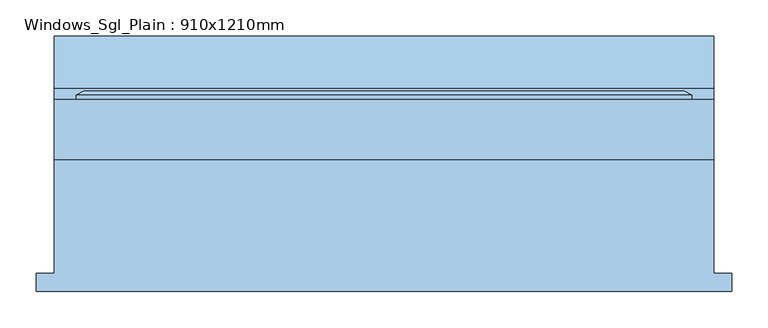
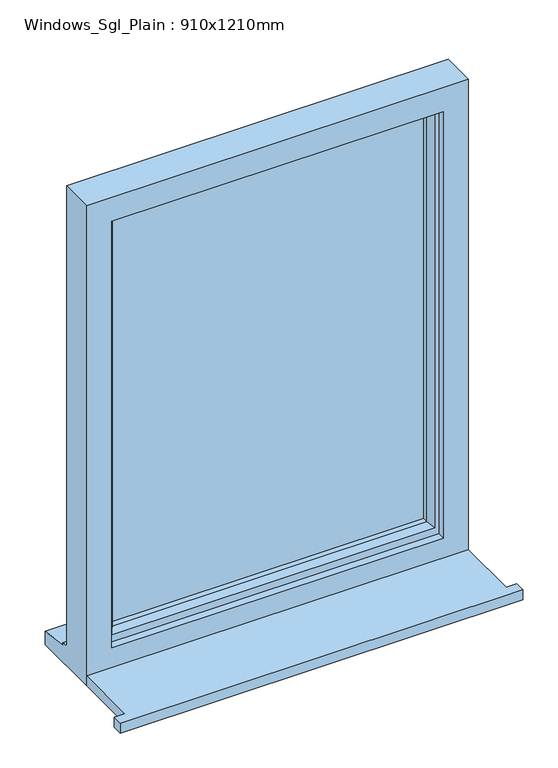
"""IFC4 building model written with IfcOpenShell, lengths in millimetres: window geometry, Windows_Sgl_Plain : 910x1210mm."""

import ifcopenshell
import ifcopenshell.guid

model = None  # the IFC model being written
_history = None  # IfcOwnerHistory: only IFC2X3 demands one
_inside = {}  # id of a spatial element -> (the spatial element, [elements in it])
_under = {}  # id of a project, library or spatial element -> (it, [spatial elements below it])
_declared = {}  # id of a project -> (the project, [libraries it declares])
_typed = {}  # id of a type object -> (the type object, [elements of that type])
_made_of = {}  # id of a material, layer set ... -> (it, [elements and type objects made of it])


def new_model(schema):
    """Start an empty IFC model of exactly this schema.

    Asked for "IFC4X3", IfcOpenShell would pick the latest addendum, in which some entities
    have other attributes; the version numbers below select the first issue.
    IFC2X3 requires an IfcOwnerHistory on every rooted entity: one is made here for all.
    """
    global model, _history
    if schema == "IFC4X3":
        model = ifcopenshell.file(schema_version=(4, 3, 0, 0))
    else:
        model = ifcopenshell.file(schema=schema)
    _inside.clear()
    _under.clear()
    _declared.clear()
    _typed.clear()
    _made_of.clear()
    _history = None
    if model.schema == "IFC2X3":
        org = make("IfcOrganization", Name="unknown")
        user = make(
            "IfcPersonAndOrganization",
            ThePerson=make("IfcPerson", FamilyName="unknown"),
            TheOrganization=org,
        )
        app = make(
            "IfcApplication",
            ApplicationDeveloper=org,
            Version="unknown",
            ApplicationFullName="unknown",
            ApplicationIdentifier="unknown",
        )
        _history = make(
            "IfcOwnerHistory",
            OwningUser=user,
            OwningApplication=app,
            ChangeAction="ADDED",
            CreationDate=0,
        )
    return model


def make(cls, **values):
    """One entity of the class cls with the attributes given. An attribute that is None is left unset."""
    return model.create_entity(
        cls, **{name: value for name, value in values.items() if value is not None}
    )


def rooted(cls, **values):
    """An entity with a GlobalId (a new one), such as an element, a storey or a relation."""
    return make(cls, GlobalId=ifcopenshell.guid.new(), OwnerHistory=_history, **values)


def si_unit(unit_type, name, prefix=None):
    """IfcSIUnit, for example si_unit("LENGTHUNIT", "METRE", prefix="MILLI")."""
    return make("IfcSIUnit", UnitType=unit_type, Prefix=prefix, Name=name)


def assignment(units):
    """IfcUnitAssignment: the units of a project."""
    return None if units is None else make("IfcUnitAssignment", Units=units)


def point(xyz):
    """IfcCartesianPoint."""
    return None if xyz is None else make("IfcCartesianPoint", Coordinates=xyz)


def direction(xyz):
    """IfcDirection."""
    return None if xyz is None else make("IfcDirection", DirectionRatios=xyz)


def frame(location, z_axis=None, x_axis=None):
    """IfcAxis2Placement3D, a coordinate frame: its origin and axes. An axis left out is left unset."""
    return make(
        "IfcAxis2Placement3D",
        Location=point(location),
        Axis=direction(z_axis),
        RefDirection=direction(x_axis),
    )


def origin():
    """The frame at (0, 0, 0) with its axes left unset."""
    return frame((0.0, 0.0, 0.0))


def place(relative_to, where):
    """IfcLocalPlacement: puts the frame where relative to a parent placement (None: the world)."""
    return make(
        "IfcLocalPlacement", PlacementRelTo=relative_to, RelativePlacement=where
    )


def context(
    kind, dimensions, precision=None, world=None, true_north=None, identifier=None
):
    """IfcGeometricRepresentationContext, for example the 3D "Model" context."""
    return make(
        "IfcGeometricRepresentationContext",
        ContextIdentifier=identifier,
        ContextType=kind,
        CoordinateSpaceDimension=dimensions,
        Precision=precision,
        WorldCoordinateSystem=world,
        TrueNorth=true_north,
    )


def project(units=None, contexts=None):
    """IfcProject with its units and contexts."""
    return rooted(
        "IfcProject",
        Name="project",
        RepresentationContexts=contexts,
        UnitsInContext=assignment(units),
    )


def spatial(cls, under=None, at=None, **own):
    """A site, building, storey or space (cls), placed at a placement, below another one or the project."""
    s = rooted(cls, ObjectPlacement=at, **own)
    if under is not None:
        _under.setdefault(under.id(), (under, []))[1].append(s)
    return s


def polyline(points):
    """IfcPolyline through the points."""
    return make("IfcPolyline", Points=[point(p) for p in points])


def outline(outer, holes=None, kind="AREA"):
    """IfcArbitraryClosedProfileDef: a profile drawn as a closed curve; with holes, ...WithVoids."""
    if holes is None:
        return make("IfcArbitraryClosedProfileDef", ProfileType=kind, OuterCurve=outer)
    return make(
        "IfcArbitraryProfileDefWithVoids",
        ProfileType=kind,
        OuterCurve=outer,
        InnerCurves=holes,
    )


def extrude(swept, where, along, depth):
    """IfcExtrudedAreaSolid: the profile swept, set in the frame where, extruded along a direction by depth."""
    return make(
        "IfcExtrudedAreaSolid",
        SweptArea=swept,
        Position=where,
        ExtrudedDirection=direction(along),
        Depth=depth,
    )


def faces_of(points, faces, orient=None, outer=None):
    """IfcFace entities. A face is a list of loops; a loop is a list of indices into points, from 0.

    orient and outer hold one flag for each loop. By default every Orientation is true, the
    first loop of a face is its IfcFaceOuterBound and the others are IfcFaceBound.
    """
    made = []
    for i, loops in enumerate(faces):
        bounds = []
        for j, loop in enumerate(loops):
            is_outer = j == 0 if outer is None else outer[i][j]
            bounds.append(
                make(
                    "IfcFaceOuterBound" if is_outer else "IfcFaceBound",
                    Bound=make("IfcPolyLoop", Polygon=[points[k] for k in loop]),
                    Orientation=True if orient is None else orient[i][j],
                )
            )
        made.append(make("IfcFace", Bounds=bounds))
    return made


def faceted_brep(points, faces, orient=None, outer=None, voids=None):
    """IfcFacetedBrep: a solid bounded by flat faces; with voids (closed shells), ...WithVoids."""
    shared = [point(p) for p in points]
    hull = make("IfcClosedShell", CfsFaces=faces_of(shared, faces, orient, outer))
    if voids is None:
        return make("IfcFacetedBrep", Outer=hull)
    return make(
        "IfcFacetedBrepWithVoids",
        Outer=hull,
        Voids=[
            make(cls, CfsFaces=faces_of(shared, fs, o, b)) for cls, fs, o, b in voids
        ],
    )


def shape(context_of_items, identifier, shape_type, items):
    """IfcShapeRepresentation: the items that make up one representation, for example the "Body"."""
    return make(
        "IfcShapeRepresentation",
        ContextOfItems=context_of_items,
        RepresentationIdentifier=identifier,
        RepresentationType=shape_type,
        Items=items,
    )


def source(mapping_origin, context_of_items, identifier, shape_type, items):
    """IfcRepresentationMap: a shape defined once, which mapped items show again and again."""
    return make(
        "IfcRepresentationMap",
        MappingOrigin=mapping_origin,
        MappedRepresentation=shape(context_of_items, identifier, shape_type, items),
    )


def transform(
    local_origin,
    x_axis=None,
    y_axis=None,
    z_axis=None,
    scale=None,
    scale2=None,
    scale3=None,
    uniform=True,
):
    """IfcCartesianTransformationOperator3D, or its non-uniform kind. x_axis, y_axis, z_axis: its Axis1, 2, 3."""
    if uniform:
        return make(
            "IfcCartesianTransformationOperator3D",
            Axis1=direction(x_axis),
            Axis2=direction(y_axis),
            LocalOrigin=point(local_origin),
            Scale=scale,
            Axis3=direction(z_axis),
        )
    return make(
        "IfcCartesianTransformationOperator3DnonUniform",
        Axis1=direction(x_axis),
        Axis2=direction(y_axis),
        LocalOrigin=point(local_origin),
        Scale=scale,
        Axis3=direction(z_axis),
        Scale2=scale2,
        Scale3=scale3,
    )


def mapped(mapping_source, mapping_target):
    """IfcMappedItem: shows the shape of a source again, moved by a transform."""
    return make(
        "IfcMappedItem", MappingSource=mapping_source, MappingTarget=mapping_target
    )


def made_of(thing, what):
    """Note that an element or type object is made of a material, layer set ...; save() writes the relation."""
    if what is not None:
        _made_of.setdefault(what.id(), (what, []))[1].append(thing)
    return thing


def element(
    cls,
    number,
    at=None,
    inside=None,
    cuts=None,
    type_object=None,
    material=None,
    context=None,
    identifier="Body",
    shape_type=None,
    held_by="IfcProductDefinitionShape",
    body=None,
    shapes=None,
    **own,
):
    """One element of the class cls, such as IfcWall. Its Tag is "e" and its number.

    at: its placement. inside: the storey or other place that contains it. cuts: it is an
    opening in that element (IfcRelVoidsElement). A single representation is given by context,
    identifier, shape_type and body (its items); several are given by shapes. held_by: the class
    of the entity that holds the representations. save() writes the other relations.
    """
    e = rooted(cls, Tag="e%d" % number, ObjectPlacement=at, **own)
    if body is not None:
        shapes = [shape(context, identifier, shape_type, body)]
    if shapes is not None:
        e.Representation = make(held_by, Representations=shapes)
    if inside is not None:
        _inside.setdefault(inside.id(), (inside, []))[1].append(e)
    if cuts is not None:
        rooted(
            "IfcRelVoidsElement", RelatingBuildingElement=cuts, RelatedOpeningElement=e
        )
    if type_object is not None:
        _typed.setdefault(type_object.id(), (type_object, []))[1].append(e)
    return made_of(e, material)


def aggregate(whole, parts):
    """IfcRelAggregates: a whole, such as a stair, and the parts it consists of."""
    return rooted("IfcRelAggregates", RelatingObject=whole, RelatedObjects=parts)


def save(model, path):
    """Write the relations noted so far, then the file.

    IfcRelAggregates (storeys below a building ...), IfcRelContainedInSpatialStructure (elements
    in a storey), IfcRelDefinesByType, IfcRelAssociatesMaterial and IfcRelDeclares: one each for
    every whole, place, type object, material and project.
    """
    for whole, parts in _under.values():
        aggregate(whole, parts)
    for where, things in _inside.values():
        rooted(
            "IfcRelContainedInSpatialStructure",
            RelatedElements=things,
            RelatingStructure=where,
        )
    for kind, things in _typed.values():
        rooted("IfcRelDefinesByType", RelatedObjects=things, RelatingType=kind)
    for what, things in _made_of.values():
        rooted("IfcRelAssociatesMaterial", RelatedObjects=things, RelatingMaterial=what)
    for by, libraries in _declared.values():
        rooted("IfcRelDeclares", RelatingContext=by, RelatedDefinitions=libraries)
    model.write(path)


def windows_sgl_plain_910x1210mm_58c8e711(model_context):
    return source(origin(), model_context, "Body", "SolidModel", [
        extrude(outline(polyline([(-480.0, -161.5434322), (-480.0, -136.5434322), (-455.0, -136.5434322), (-455.0, 20.4565678), (455.0, 20.4565678), (455.0, -136.5434322), (480.0, -136.5434322), (480.0, -161.5434322), (-480.0, -161.5434322)])), frame((0.0, 0.0, 900.0), z_axis=(0.0, 0.0, 1.0), x_axis=(1.0, 0.0, 0.0)), (0.0, 0.0, 1.0), 25.0),
        faceted_brep([(-455.0, 20.4565678, 900.0), (455.0, 20.4565678, 900.0), (455.0, 20.4565678, 2110.0), (-455.0, 20.4565678, 2110.0), (-395.0, 20.4565678, 2050.0), (395.0, 20.4565678, 2050.0), (395.0, 20.4565678, 975.0), (-395.0, 20.4565678, 975.0), (-455.0, 103.4565678, 2110.0), (-455.0, 103.4565678, 951.0), (-455.0, 118.4565678, 949.68767), (-455.0, 118.4565678, 944.7449676), (-455.0, 190.9565678, 933.8088847), (-455.0, 190.9565678, 900.0), (455.0, 103.4565678, 2110.0), (455.0, 103.4565678, 951.0), (-415.0, 103.4565678, 2070.0), (-415.0, 103.4565678, 963.0), (415.0, 103.4565678, 963.0), (415.0, 103.4565678, 2070.0), (-415.0, 38.4565678, 2070.0), (-415.0, 38.4565678, 963.0), (415.0, 38.4565678, 2070.0), (415.0, 38.4565678, 963.0), (-395.0, 38.4565678, 2050.0), (-395.0, 38.4565678, 975.0), (395.0, 38.4565678, 975.0), (395.0, 38.4565678, 2050.0), (455.0, 190.9565678, 900.0), (455.0, 190.9565678, 933.8088847), (455.0, 118.4565678, 944.7449676), (455.0, 118.4565678, 949.68767)], [[[0, 1, 2, 3], [4, 5, 6, 7]], [[0, 3, 8, 9, 10, 11, 12, 13]], [[9, 8, 14, 15], [16, 17, 18, 19]], [[17, 16, 20, 21]], [[20, 22, 23, 21], [24, 25, 26, 27]], [[24, 4, 7, 25]], [[3, 2, 14, 8]], [[16, 19, 22, 20]], [[5, 4, 24, 27]], [[15, 14, 2, 1, 28, 29, 30, 31]], [[19, 18, 23, 22]], [[5, 27, 26, 6]], [[28, 1, 0, 13]], [[29, 28, 13, 12]], [[30, 29, 12, 11]], [[31, 30, 11, 10]], [[15, 31, 10, 9]], [[21, 23, 18, 17]], [[7, 6, 26, 25]]]),
        extrude(outline(polyline([(385.0, 67.4565678), (-385.0, 67.4565678), (-385.0, 91.4565678), (385.0, 91.4565678), (385.0, 67.4565678)])), frame((0.0, 0.0, 993.0), z_axis=(0.0, 0.0, 1.0), x_axis=(1.0, 0.0, 0.0)), (0.0, 0.0, 1.0), 1047.0),
        faceted_brep([(-425.0, 103.4565678, 2080.0), (-425.0, 109.2300705, 2080.0), (-425.0, 109.2300705, 953.0), (-425.0, 103.4565678, 953.0), (-415.0, 38.4565678, 2070.0), (-415.0, 103.4565678, 2070.0), (-415.0, 103.4565678, 963.0), (-415.0, 38.4565678, 963.0), (-375.0, 52.9494677, 2030.0), (-385.1480377, 38.4565678, 2040.1480377), (-385.1480377, 38.4565678, 992.8519623), (-375.0, 52.9494677, 1003.0), (-375.0, 67.4565678, 2030.0), (-375.0, 67.4565678, 1003.0), (-385.0, 91.4565678, 2040.0), (-385.0, 67.4565678, 2040.0), (-385.0, 67.4565678, 993.0), (-385.0, 91.4565678, 993.0), (-375.0, 109.2300705, 2030.0), (-375.0, 91.4565678, 2030.0), (-375.0, 91.4565678, 1003.0), (-375.0, 109.2300705, 1003.0), (-392.4457548, 115.0035732, 2047.4457548), (-392.4457548, 115.0035732, 985.5542452), (-414.2153903, 115.0035732, 2069.2153903), (-414.2153903, 115.0035732, 963.7846097), (425.0, 109.2300705, 953.0), (425.0, 103.4565678, 953.0), (415.0, 103.4565678, 963.0), (415.0, 38.4565678, 963.0), (385.1480377, 38.4565678, 992.8519623), (375.0, 52.9494677, 1003.0), (375.0, 67.4565678, 1003.0), (385.0, 67.4565678, 993.0), (385.0, 91.4565678, 993.0), (375.0, 91.4565678, 1003.0), (375.0, 109.2300705, 1003.0), (392.4457548, 115.0035732, 985.5542452), (414.2153903, 115.0035732, 963.7846097), (425.0, 109.2300705, 2080.0), (425.0, 103.4565678, 2080.0), (415.0, 103.4565678, 2070.0), (415.0, 38.4565678, 2070.0), (385.1480377, 38.4565678, 2040.1480377), (375.0, 52.9494677, 2030.0), (375.0, 67.4565678, 2030.0), (385.0, 67.4565678, 2040.0), (385.0, 91.4565678, 2040.0), (375.0, 91.4565678, 2030.0), (375.0, 109.2300705, 2030.0), (392.4457548, 115.0035732, 2047.4457548), (414.2153903, 115.0035732, 2069.2153903)], [[[0, 1, 2, 3]], [[4, 5, 6, 7]], [[8, 9, 10, 11]], [[12, 8, 11, 13]], [[14, 15, 16, 17]], [[18, 19, 20, 21]], [[22, 18, 21, 23]], [[1, 24, 25, 2]], [[3, 2, 26, 27]], [[7, 6, 28, 29]], [[11, 10, 30, 31]], [[13, 11, 31, 32]], [[17, 16, 33, 34]], [[21, 20, 35, 36]], [[23, 21, 36, 37]], [[2, 25, 38, 26]], [[27, 26, 39, 40]], [[29, 28, 41, 42]], [[31, 30, 43, 44]], [[32, 31, 44, 45]], [[34, 33, 46, 47]], [[36, 35, 48, 49]], [[37, 36, 49, 50]], [[26, 38, 51, 39]], [[40, 39, 1, 0]], [[3, 27, 40, 0], [5, 41, 28, 6]], [[42, 41, 5, 4]], [[7, 29, 42, 4], [9, 43, 30, 10]], [[44, 43, 9, 8]], [[45, 44, 8, 12]], [[15, 46, 33, 16], [13, 32, 45, 12]], [[47, 46, 15, 14]], [[17, 34, 47, 14], [19, 48, 35, 20]], [[49, 48, 19, 18]], [[50, 49, 18, 22]], [[24, 51, 38, 25], [23, 37, 50, 22]], [[39, 51, 24, 1]]]),
    ])


if __name__ == "__main__":
    model = new_model("IFC4")
    model_context = context("Model", 3, world=origin())
    ifc_project = project(units=[si_unit("LENGTHUNIT", "METRE", prefix="MILLI")], contexts=[model_context])
    site = spatial("IfcSite", under=ifc_project)
    building = spatial("IfcBuilding", under=site)
    placement = place(None, origin())
    windows_sgl_plain_910x1210mm_shape = windows_sgl_plain_910x1210mm_58c8e711(model_context)
    element("IfcWindow", 1, ObjectType="Windows_Sgl_Plain : 910x1210mm", at=placement, inside=building, context=model_context, shape_type="MappedRepresentation", body=[
        mapped(windows_sgl_plain_910x1210mm_shape, transform((0.0, 0.0, 0.0), x_axis=(1.0, 0.0, 0.0), y_axis=(0.0, 1.0, 0.0), z_axis=(0.0, 0.0, 1.0))),
    ])
    save(model, "model.ifc")

# Revit data of these elements
# Type "Windows_Sgl_Plain : 910x1210mm"
#   Type Mark = "45"
#   Operation = "SinglePanel"
#   Construction Type Id = "SGL"
#   Manufacturer = "Revit"
#   Keynote = "L10"
#   Analytic Construction = "Large single-glazed windows"
#   Wrap Layers (Ext) from Ext = 102.5 mm
#   Wrap Layers (Int) from Ext = 177.5 mm
#   Window Board Projection = 25 mm
#   Window Board Extension = 25 mm
#   Visual Light Transmittance = 0.9
#   Solar Heat Gain Coefficient = 0.86
#   Rough Width = 910 mm
#   Rough Height = 1210 mm
#   Height = 1210 mm
#   Width = 910 mm
#   Heat Transfer Coefficient (U) = 5.5617 W/(m²·K)
#   Glazing Thickness = 24 mm
#   FrameOffset - External = 50 mm
#   Frame Depth = 65 mm
#   Default Head Height = 2110 mm
#   Cill Depth = 87.5 mm
#   Cavity Closer Width = 50 mm
#   Cavity Closer Offset from Ext = 102.5 mm
#   Cavity Closer Depth = 85 mm
#   Define Thermal Properties by = 1
#   Vis - Cavity Closers = yes
#   Define Thermal Properties by = 1
#   Material Trim = Window Frame
#   Material Glass = Glass
#   Material Frame = Window Frame
#   Wall Closure = (empty or 0)
# Element 1 (IfcWindow, "Windows_Sgl_Plain : 910x1210mm")
#   Materials on its faces: "Window Frame", "Glass"
# Materials
#   "Window Frame": class "Miscellaneous", colour RGB 249 249 249, transparency 0, Keynote = "L10", Cost = 0
#   "Glass": class "Glass", colour RGB 0 128 192, transparency 0.9, Description = "Soda Lime Glass", Cost = 0
